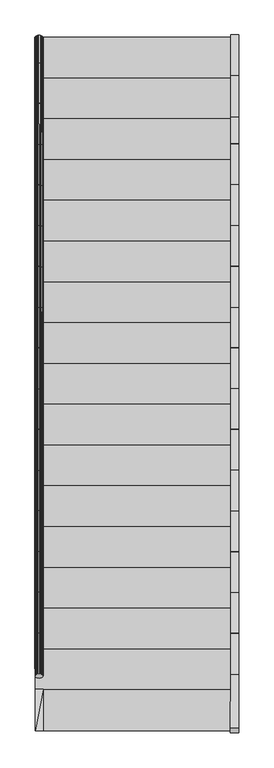
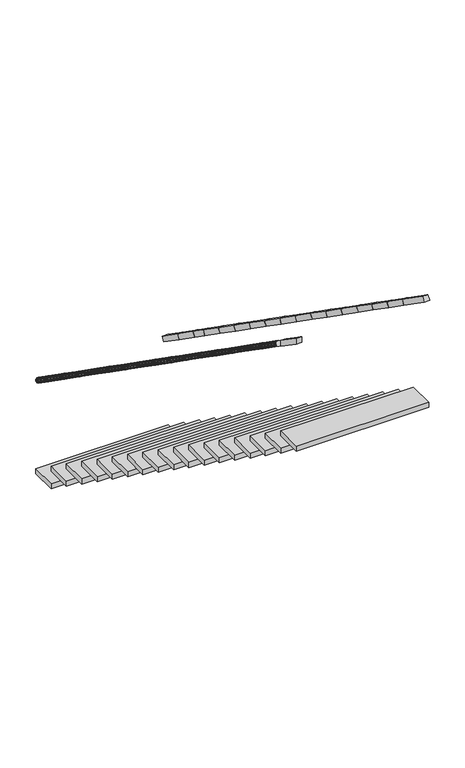
"""IFC4 building model written with IfcOpenShell, lengths in millimetres: stair geometry, 0_3d."""

from ifc_helpers import new_model, si_unit, frame, origin, origin_with_axes, place, context, project, spatial, polyline, outline, extrude, faceted_brep, source, transform, mapped, element, save


def stair_a708374c(model_context):
    return source(origin(), model_context, "Body", "SolidModel", [
        extrude(outline(polyline([(1249.4490496, 514.5019196), (1249.4123204, 264.3787636), (0.5876783, 268.1325506), (0.5509483, 518.0098269), (1249.4490496, 514.5019196)])), frame((0.0, 0.0, 2625.0), z_axis=(0.0, 0.0, 1.0), x_axis=(1.0, 0.0, 0.0)), (0.0, 0.0, 1.0), 50.0),
        extrude(outline(polyline([(8.0820225, -49.3424858), (0.0, 0.0), (301.2464918, 49.3424859), (309.3285142, 1e-07), (8.0820225, -49.3424858)])), frame((1249.9611524, 4001.8916658, 1074.5520464), z_axis=(8.41828832501973e-05, 0.5732803649279318, 0.8193592716881524), x_axis=(-0.1617591834181913, -0.8085607212194018, 0.5657415723464564)), (0.0, 0.0, 1.0), 50.0),
        faceted_brep([(1.4325369, 2844.6597545, 1907.7450176), (0.2083434, 2848.7849185, 1913.6355824), (1.4313241, 2852.9104422, 1919.5261472), (4.9817651, 2856.6324906, 1924.8401024), (10.5121244, 2859.5867237, 1929.0572812), (17.4810521, 2861.4839606, 1931.7648767), (25.2063808, 2862.1384864, 1932.6978505), (32.9319016, 2861.4862317, 1931.7648767), (39.9013867, 2859.5910437, 1929.0572812), (45.4326143, 2856.6384366, 1924.8401024), (48.9841494, 2852.9174321, 1919.5261472), (50.2083429, 2848.7922681, 1913.6355824), (48.9853622, 2844.6667444, 1907.7450176), (45.4349212, 2840.944696, 1902.4310623), (39.9045618, 2837.9904629, 1898.2138835), (32.9356342, 2836.093226, 1895.5062881), (25.2103054, 2835.4387002, 1894.5733142), (17.4847846, 2836.0909549, 1895.5062881), (10.5152995, 2837.9861429, 1898.2138835), (4.9840719, 2840.9387501, 1902.4310623), (0.245074, 2598.9029786, 2088.6355868), (1.4680547, 2603.028502, 2094.5261518), (5.0184957, 2606.7505501, 2099.8401073), (10.548855, 2609.704783, 2104.0572862), (17.5177827, 2611.6020197, 2106.7648818), (25.2431114, 2612.2565455, 2107.6978556), (32.9686322, 2611.6042908, 2106.7648818), (39.9381173, 2609.709103, 2104.0572862), (45.4693449, 2606.7564961, 2099.8401073), (49.02088, 2603.0354919, 2094.5261518), (50.2450735, 2598.9103282, 2088.6355868), (49.0220928, 2594.7848048, 2082.7450218), (45.4716518, 2591.0627567, 2077.4310663), (39.9412924, 2588.1085238, 2073.2138874), (32.9723648, 2586.2112871, 2070.5062918), (25.2470361, 2585.5567613, 2069.573318), (17.5215152, 2586.209016, 2070.5062918), (10.5520301, 2588.1042038, 2073.2138874), (5.0208025, 2591.0568107, 2077.4310663), (1.4692675, 2594.7778149, 2082.7450218)], [[[0, 1, 2, 3, 4, 5, 6, 7, 8, 9, 10, 11, 12, 13, 14, 15, 16, 17, 18, 19]], [[2, 1, 20, 21]], [[3, 2, 21, 22]], [[4, 3, 22, 23]], [[5, 4, 23, 24]], [[6, 5, 24, 25]], [[7, 6, 25, 26]], [[8, 7, 26, 27]], [[9, 8, 27, 28]], [[10, 9, 28, 29]], [[11, 10, 29, 30]], [[12, 11, 30, 31]], [[13, 12, 31, 32]], [[14, 13, 32, 33]], [[15, 14, 33, 34]], [[16, 15, 34, 35]], [[17, 16, 35, 36]], [[18, 17, 36, 37]], [[19, 18, 37, 38]], [[0, 19, 38, 39]], [[1, 0, 39, 20]], [[21, 20, 39, 38, 37, 36, 35, 34, 33, 32, 31, 30, 29, 28, 27, 26, 25, 24, 23, 22]]]),
        extrude(outline(polyline([(1249.5225078, 1014.7482313), (1249.4857787, 764.6250755), (0.5142184, 767.8870744), (0.4774885, 1017.7642932), (1249.5225078, 1014.7482313)])), frame((0.0, 0.0, 2275.0), z_axis=(0.0, 0.0, 1.0), x_axis=(1.0, 0.0, 0.0)), (0.0, 0.0, 1.0), 50.0),
        faceted_brep([(1.4692675, 2594.7778149, 2082.7450218), (0.245074, 2598.9029786, 2088.6355868), (1.4680547, 2603.028502, 2094.5261518), (5.0184957, 2606.7505501, 2099.8401073), (10.548855, 2609.704783, 2104.0572862), (17.5177827, 2611.6020197, 2106.7648818), (25.2431114, 2612.2565455, 2107.6978556), (32.9686322, 2611.6042908, 2106.7648818), (39.9381173, 2609.709103, 2104.0572862), (45.4693449, 2606.7564961, 2099.8401073), (49.02088, 2603.0354919, 2094.5261518), (50.2450735, 2598.9103282, 2088.6355868), (49.0220928, 2594.7848048, 2082.7450218), (45.4716518, 2591.0627567, 2077.4310663), (39.9412924, 2588.1085238, 2073.2138874), (32.9723648, 2586.2112871, 2070.5062918), (25.2470361, 2585.5567613, 2069.573318), (17.5215152, 2586.209016, 2070.5062918), (10.5520301, 2588.1042038, 2073.2138874), (5.0208025, 2591.0568107, 2077.4310663), (0.2818046, 2349.0210098, 2263.6355913), (1.5047853, 2353.1465328, 2269.5261565), (5.0552263, 2356.8685807, 2274.8401122), (10.5855856, 2359.8228133, 2279.0572913), (17.5545133, 2361.7200499, 2281.7648869), (25.279842, 2362.3745756, 2282.6978608), (33.0053628, 2361.722321, 2281.7648869), (39.9748479, 2359.8271333, 2279.0572913), (45.5060756, 2356.8745266, 2274.8401122), (49.0576106, 2353.1535227, 2269.5261565), (50.2818041, 2349.0283594, 2263.6355913), (49.0588234, 2344.9028363, 2257.745026), (45.5083824, 2341.1807885, 2252.4310703), (39.978023, 2338.2265558, 2248.2138912), (33.0090954, 2336.3293193, 2245.5062956), (25.2837667, 2335.6747935, 2244.5733217), (17.5582459, 2336.3270481, 2245.5062956), (10.5887608, 2338.2222359, 2248.2138912), (5.0575331, 2341.1748425, 2252.4310703), (1.5059981, 2344.8958464, 2257.745026)], [[[0, 1, 2, 3, 4, 5, 6, 7, 8, 9, 10, 11, 12, 13, 14, 15, 16, 17, 18, 19]], [[2, 1, 20, 21]], [[3, 2, 21, 22]], [[4, 3, 22, 23]], [[5, 4, 23, 24]], [[6, 5, 24, 25]], [[7, 6, 25, 26]], [[8, 7, 26, 27]], [[9, 8, 27, 28]], [[10, 9, 28, 29]], [[11, 10, 29, 30]], [[12, 11, 30, 31]], [[13, 12, 31, 32]], [[14, 13, 32, 33]], [[15, 14, 33, 34]], [[16, 15, 34, 35]], [[17, 16, 35, 36]], [[18, 17, 36, 37]], [[19, 18, 37, 38]], [[0, 19, 38, 39]], [[1, 0, 39, 20]], [[21, 20, 39, 38, 37, 36, 35, 34, 33, 32, 31, 30, 29, 28, 27, 26, 25, 24, 23, 22]]]),
        extrude(outline(polyline([(8.0820225, -49.3424858), (0.0, 0.0), (301.2464919, 49.3424859), (309.3285143, 1e-07), (8.0820225, -49.3424858)])), frame((1249.7895422, 2833.2364482, 1892.2240093), z_axis=(8.418288334449686e-05, 0.5732803647665086, 0.8193592718010952), x_axis=(-0.16175918336906983, -0.8085607213374504, 0.5657415721917858)), (0.0, 0.0, 1.0), 50.0),
        extrude(outline(polyline([(8.0820225, -49.3424859), (0.0, 0.0), (301.246492, 49.3424859), (309.3285144, 0.0), (8.0820225, -49.3424859)])), frame((1249.679357, 2082.8817614, 2417.2240094), z_axis=(8.418288319098076e-05, 0.5732803645012542, 0.8193592719866855), x_axis=(-0.16175918329309924, -0.8085607215308216, 0.5657415719371407)), (0.0, 0.0, 1.0), 50.0),
        extrude(outline(polyline([(8.0820225, -49.3424859), (0.0, 0.0), (301.2464924, 49.3424859), (309.3285148, 0.0), (8.0820225, -49.3424859)])), frame((1249.495715, 832.2906153, 3292.2240094), z_axis=(8.418288310454991e-05, 0.5732803637766174, 0.8193592724936917), x_axis=(-0.16175918308892365, -0.8085607220586004, 0.565741571241215)), (0.0, 0.0, 1.0), 50.0),
        extrude(outline(polyline([(1249.6326952, 1765.1176979), (1249.5959661, 1514.9945425), (0.4040287, 1517.5186441), (0.3672988, 1767.3957763), (1249.6326952, 1765.1176979)])), frame((0.0, 0.0, 1750.0), z_axis=(0.0, 0.0, 1.0), x_axis=(1.0, 0.0, 0.0)), (0.0, 0.0, 1.0), 50.0),
        faceted_brep([(1.3958063, 3094.5416652, 1732.7450133), (0.1716128, 3098.6668296, 1738.6355779), (1.3945935, 3102.7923536, 1744.5261425), (4.9450345, 3106.5144023, 1749.8400975), (10.4753938, 3109.4686356, 1754.0572762), (17.4443215, 3111.3658726, 1756.7648715), (25.1696502, 3112.0203985, 1757.6978453), (32.895171, 3111.3681438, 1756.7648715), (39.8646561, 3109.4729556, 1754.0572762), (45.3958837, 3106.5203482, 1749.8400975), (48.9474188, 3102.7993435, 1744.5261425), (50.1716122, 3098.6741791, 1738.6355779), (48.9486316, 3094.5486551, 1732.7450133), (45.3981906, 3090.8266064, 1727.4310583), (39.8678312, 3087.8723731, 1723.2138796), (32.8989036, 3085.9751361, 1720.5062843), (25.1735748, 3085.3206102, 1719.5733105), (17.448054, 3085.9728649, 1720.5062843), (10.4785689, 3087.8680531, 1723.2138796), (4.9473413, 3090.8206605, 1727.4310583), (0.2083434, 2848.7849185, 1913.6355824), (1.4313241, 2852.9104422, 1919.5261472), (4.9817651, 2856.6324906, 1924.8401024), (10.5121244, 2859.5867237, 1929.0572812), (17.4810521, 2861.4839606, 1931.7648767), (25.2063808, 2862.1384864, 1932.6978505), (32.9319016, 2861.4862317, 1931.7648767), (39.9013867, 2859.5910437, 1929.0572812), (45.4326143, 2856.6384366, 1924.8401024), (48.9841494, 2852.9174321, 1919.5261472), (50.2083429, 2848.7922681, 1913.6355824), (48.9853622, 2844.6667444, 1907.7450176), (45.4349212, 2840.944696, 1902.4310623), (39.9045618, 2837.9904629, 1898.2138835), (32.9356342, 2836.093226, 1895.5062881), (25.2103054, 2835.4387002, 1894.5733142), (17.4847846, 2836.0909549, 1895.5062881), (10.5152995, 2837.9861429, 1898.2138835), (4.9840719, 2840.9387501, 1902.4310623), (1.4325369, 2844.6597545, 1907.7450176)], [[[0, 1, 2, 3, 4, 5, 6, 7, 8, 9, 10, 11, 12, 13, 14, 15, 16, 17, 18, 19]], [[2, 1, 20, 21]], [[3, 2, 21, 22]], [[4, 3, 22, 23]], [[5, 4, 23, 24]], [[6, 5, 24, 25]], [[7, 6, 25, 26]], [[8, 7, 26, 27]], [[9, 8, 27, 28]], [[10, 9, 28, 29]], [[11, 10, 29, 30]], [[12, 11, 30, 31]], [[13, 12, 31, 32]], [[14, 13, 32, 33]], [[15, 14, 33, 34]], [[16, 15, 34, 35]], [[17, 16, 35, 36]], [[18, 17, 36, 37]], [[19, 18, 37, 38]], [[0, 19, 38, 39]], [[1, 0, 39, 20]], [[21, 20, 39, 38, 37, 36, 35, 34, 33, 32, 31, 30, 29, 28, 27, 26, 25, 24, 23, 22]]]),
        extrude(outline(polyline([(1249.7061535, 2265.3640086), (1249.6694243, 2015.2408533), (0.3305689, 2017.2728797), (0.293839, 2267.1499541), (1249.7061535, 2265.3640086)])), frame((0.0, 0.0, 1400.0), z_axis=(0.0, 0.0, 1.0), x_axis=(1.0, 0.0, 0.0)), (0.0, 0.0, 1.0), 50.0),
        faceted_brep([(1.7263819, 845.6034293, 3307.7450513), (0.5021884, 849.7285907, 3313.6356179), (1.7251691, 853.8541119, 3319.5261845), (5.27561, 857.576158, 3324.8401414), (10.8059694, 860.5303893, 3329.0573215), (17.7748971, 862.4276249, 3331.7649177), (25.5002258, 863.0821504, 3332.6978918), (33.2257466, 862.4298961, 3331.7649177), (40.1952317, 860.5347092, 3329.0573215), (45.7264593, 857.5821039, 3324.8401414), (49.2779944, 853.8611018, 3319.5261845), (50.5021878, 849.7359403, 3313.6356179), (49.2792072, 845.6104192, 3307.7450513), (45.7287662, 841.8883731, 3302.4310944), (40.1984068, 838.9341418, 3298.2139144), (33.2294792, 837.0369061, 3295.5063181), (25.5041504, 836.3823807, 3294.573344), (17.7786296, 837.034635, 3295.5063181), (10.8091445, 838.9298218, 3298.2139144), (5.2779169, 841.8824271, 3302.4310944), (0.538919, 599.84642, 3488.6356224), (1.7618997, 603.9719408, 3494.5261892), (5.3123407, 607.6939866, 3499.8401463), (10.8427001, 610.6482177, 3504.0573265), (17.8116277, 612.5454532, 3506.7649229), (25.5369564, 613.1999786, 3507.697897), (33.2624772, 612.5477243, 3506.7649229), (40.2319623, 610.6525376, 3504.0573265), (45.76319, 607.6999326, 3499.8401463), (49.314725, 603.9789307, 3494.5261892), (50.5389185, 599.8537696, 3488.6356224), (49.3159378, 595.7282487, 3482.7450556), (45.7654968, 592.0062029, 3477.4310985), (40.2351375, 589.0519719, 3473.2139182), (33.2662098, 587.1547364, 3470.5063219), (25.5408811, 586.500211, 3469.5733477), (17.8153603, 587.1524652, 3470.5063219), (10.8458752, 589.0476519, 3473.2139182), (5.3146475, 592.000257, 3477.4310985), (1.7631125, 595.7212589, 3482.7450556)], [[[0, 1, 2, 3, 4, 5, 6, 7, 8, 9, 10, 11, 12, 13, 14, 15, 16, 17, 18, 19]], [[2, 1, 20, 21]], [[3, 2, 21, 22]], [[4, 3, 22, 23]], [[5, 4, 23, 24]], [[6, 5, 24, 25]], [[7, 6, 25, 26]], [[8, 7, 26, 27]], [[9, 8, 27, 28]], [[10, 9, 28, 29]], [[11, 10, 29, 30]], [[12, 11, 30, 31]], [[13, 12, 31, 32]], [[14, 13, 32, 33]], [[15, 14, 33, 34]], [[16, 15, 34, 35]], [[17, 16, 35, 36]], [[18, 17, 36, 37]], [[19, 18, 37, 38]], [[0, 19, 38, 39]], [[1, 0, 39, 20]], [[21, 20, 39, 38, 37, 36, 35, 34, 33, 32, 31, 30, 29, 28, 27, 26, 25, 24, 23, 22]]]),
        faceted_brep([(0.6244082, 14.2556075, 3867.0), (0.5876783, 268.1325506, 3692.0), (50.5877009, 267.9822577, 3692.0), (50.6244323, 14.2555335, 3867.0), (50.5877009, 267.9822577, 3750.0), (0.5876783, 268.1325506, 3750.0), (0.6244082, 14.2556075, 3925.0), (50.6244323, 14.2555335, 3925.0)], [[[0, 1, 2]], [[3, 0, 2]], [[4, 5, 6]], [[7, 4, 6]], [[4, 2, 1, 5]], [[5, 1, 0, 6]], [[6, 0, 3, 7]], [[7, 3, 2, 4]]]),
        extrude(outline(polyline([(8.0820224, -49.3424859), (0.0, 0.0), (301.2464922, 49.3424859), (309.3285146, 0.0), (8.0820224, -49.3424859)])), frame((1249.5691718, 1332.527074, 2942.2240094), z_axis=(8.418288311948242e-05, 0.5732803641088847, 0.8193592722612145), x_axis=(-0.16175918318212845, -0.8085607218166563, 0.5657415715603531)), (0.0, 0.0, 1.0), 50.0),
        extrude(outline(polyline([(1.2235871, -7.1914683), (0.0, 0.0), (1.2235871, 7.1914683), (4.7745752, 13.6789855), (10.3053687, 18.8275083), (17.2745752, 22.1330635), (25.0, 23.2720802), (32.7254248, 22.1330635), (39.6946313, 18.8275084), (45.2254248, 13.6789855), (48.7764129, 7.1914683), (50.0, 0.0), (48.7764129, -7.1914683), (45.2254249, -13.6789854), (39.6946313, -18.8275083), (32.7254249, -22.1330635), (25.0, -23.2720802), (17.2745751, -22.1330634), (10.3053687, -18.8275083), (4.7745751, -13.6789855), (1.2235871, -7.1914683)])), frame((0.0, 4266.1655097, 921.0), z_axis=(0.00012040167666258672, -0.8191044431453997, 0.5736443991907366), x_axis=(0.9999999891966984, 0.00014699184745837235, 0.0)), (0.0, 0.0, 1.0), 205.067042),
        extrude(outline(polyline([(1249.8897991, 3515.9797843), (1249.85307, 3265.8566293), (0.1469195, 3266.6579632), (0.1101896, 3516.5348933), (1249.8897991, 3515.9797843)])), frame((0.0, 0.0, 525.0), z_axis=(0.0, 0.0, 1.0), x_axis=(1.0, 0.0, 0.0)), (0.0, 0.0, 1.0), 50.0),
        extrude(outline(polyline([(1249.8163409, 3015.7334742), (1249.7796117, 2765.610319), (0.2203792, 2766.9040165), (0.1836493, 3016.7810043), (1249.8163409, 3015.7334742)])), frame((0.0, 0.0, 875.0), z_axis=(0.0, 0.0, 1.0), x_axis=(1.0, 0.0, 0.0)), (0.0, 0.0, 1.0), 50.0),
        extrude(outline(polyline([(1249.9999865, 4266.3492495), (1249.9632574, 4016.2260945), (0.0367299, 4016.2886665), (0.0, 4266.1655097), (1249.9999865, 4266.3492495)])), origin_with_axes(), (0.0, 0.0, 1.0), 50.0),
        faceted_brep([(1.5794593, 1845.1318228, 2607.7450345), (0.3552659, 1849.2569855, 2613.6356001), (1.5782465, 1853.3825079, 2619.5261658), (5.1286875, 1857.1045552, 2624.8401219), (10.6590469, 1860.0587874, 2629.0573013), (17.6279745, 1861.9560236, 2631.7648972), (25.3533033, 1862.6105493, 2632.6978712), (33.0788241, 1861.9582948, 2631.7648972), (40.0483092, 1860.0631074, 2629.0573013), (45.5795368, 1857.1105012, 2624.8401219), (49.1310718, 1853.3894978, 2619.5261658), (50.3552653, 1849.2643351, 2613.6356001), (49.1322846, 1845.1388127, 2607.7450345), (45.5818436, 1841.4167654, 2602.4310784), (40.0514843, 1838.4625333, 2598.213899), (33.0825566, 1836.565297, 2595.5063031), (25.3572279, 1835.9107713, 2594.5733291), (17.6317071, 1836.5630258, 2595.5063031), (10.662222, 1838.4582133, 2598.213899), (5.1309944, 1841.4108195, 2602.4310784), (0.3919965, 1599.3749301, 2788.6356046), (1.6149772, 1603.5004522, 2794.5261705), (5.1654181, 1607.2224992, 2799.8401268), (10.6957775, 1610.1767311, 2804.0573064), (17.6647052, 1612.0739672, 2806.7649023), (25.3900339, 1612.7284928, 2807.6978763), (33.1155547, 1612.0762384, 2806.7649023), (40.0850398, 1610.1810511, 2804.0573064), (45.6162674, 1607.2284451, 2799.8401268), (49.1678025, 1603.5074421, 2794.5261705), (50.3919959, 1599.3822797, 2788.6356046), (49.1690153, 1595.2567576, 2782.7450387), (45.6185743, 1591.5347106, 2777.4310824), (40.0882149, 1588.5804787, 2773.2139028), (33.1192873, 1586.6832425, 2770.5063068), (25.3939585, 1586.0287169, 2769.5733329), (17.6684377, 1586.6809714, 2770.5063068), (10.6989526, 1588.5761587, 2773.2139028), (5.167725, 1591.5287647, 2777.4310824), (1.6161899, 1595.2497677, 2782.7450387)], [[[0, 1, 2, 3, 4, 5, 6, 7, 8, 9, 10, 11, 12, 13, 14, 15, 16, 17, 18, 19]], [[2, 1, 20, 21]], [[3, 2, 21, 22]], [[4, 3, 22, 23]], [[5, 4, 23, 24]], [[6, 5, 24, 25]], [[7, 6, 25, 26]], [[8, 7, 26, 27]], [[9, 8, 27, 28]], [[10, 9, 28, 29]], [[11, 10, 29, 30]], [[12, 11, 30, 31]], [[13, 12, 31, 32]], [[14, 13, 32, 33]], [[15, 14, 33, 34]], [[16, 15, 34, 35]], [[17, 16, 35, 36]], [[18, 17, 36, 37]], [[19, 18, 37, 38]], [[0, 19, 38, 39]], [[1, 0, 39, 20]], [[21, 20, 39, 38, 37, 36, 35, 34, 33, 32, 31, 30, 29, 28, 27, 26, 25, 24, 23, 22]]]),
        faceted_brep([(1.2856145, 3844.1872239, 1207.7450006), (0.061421, 3848.3123892, 1213.6355645), (1.2844017, 3852.4379142, 1219.5261284), (4.8348427, 3856.1599637, 1224.8400829), (10.365202, 3859.1141977, 1229.057261), (17.3341297, 3861.0114352, 1231.7648561), (25.0594584, 3861.6659612, 1232.6978297), (32.7849792, 3861.0137063, 1231.7648561), (39.7544643, 3859.1185177, 1229.057261), (45.2856919, 3856.1659097, 1224.8400829), (48.837227, 3852.444904, 1219.5261284), (50.0614205, 3848.3197388, 1213.6355645), (48.8384398, 3844.1942138, 1207.7450006), (45.2879988, 3840.4721642, 1202.4310462), (39.7576394, 3837.5179302, 1198.213868), (32.7887118, 3835.6206928, 1195.506273), (25.0633831, 3834.9661667, 1194.5732993), (17.3378622, 3835.6184216, 1195.506273), (10.3683771, 3837.5136102, 1198.213868), (4.8371495, 3840.4662183, 1202.4310462), (0.0981516, 3598.4305649, 1388.635569), (1.3211323, 3602.5560896, 1394.5261331), (4.8715733, 3606.2781388, 1399.8400878), (10.4019326, 3609.2323726, 1404.0572661), (17.3708603, 3611.1296099, 1406.7648612), (25.096189, 3611.7841359, 1407.6978349), (32.8217098, 3611.1318811, 1406.7648612), (39.7911949, 3609.2366926, 1404.0572661), (45.3224225, 3606.2840848, 1399.8400878), (48.8739576, 3602.5630794, 1394.5261331), (50.0981511, 3598.4379145, 1388.635569), (48.8751704, 3594.3123898, 1382.7450049), (45.3247294, 3590.5903405, 1377.4310502), (39.79437, 3587.6361067, 1373.2138719), (32.8254424, 3585.7388695, 1370.5062768), (25.1001137, 3585.0843435, 1369.5733031), (17.3745928, 3585.7365983, 1370.5062768), (10.4051077, 3587.6317868, 1373.2138719), (4.8738801, 3590.5843946, 1377.4310502), (1.3223451, 3594.3053999, 1382.7450049)], [[[0, 1, 2, 3, 4, 5, 6, 7, 8, 9, 10, 11, 12, 13, 14, 15, 16, 17, 18, 19]], [[2, 1, 20, 21]], [[3, 2, 21, 22]], [[4, 3, 22, 23]], [[5, 4, 23, 24]], [[6, 5, 24, 25]], [[7, 6, 25, 26]], [[8, 7, 26, 27]], [[9, 8, 27, 28]], [[10, 9, 28, 29]], [[11, 10, 29, 30]], [[12, 11, 30, 31]], [[13, 12, 31, 32]], [[14, 13, 32, 33]], [[15, 14, 33, 34]], [[16, 15, 34, 35]], [[17, 16, 35, 36]], [[18, 17, 36, 37]], [[19, 18, 37, 38]], [[0, 19, 38, 39]], [[1, 0, 39, 20]], [[21, 20, 39, 38, 37, 36, 35, 34, 33, 32, 31, 30, 29, 28, 27, 26, 25, 24, 23, 22]]]),
        faceted_brep([(1.6896512, 1095.4855709, 3132.7450471), (0.4654577, 1099.6107327, 3138.6356135), (1.6884384, 1103.7362542, 3144.5261798), (5.2388794, 1107.4583006, 3149.8401365), (10.7692388, 1110.4125321, 3154.0573164), (17.7381664, 1112.3097679, 3156.7649126), (25.4634951, 1112.9642934, 3157.6978867), (33.189016, 1112.312039, 3156.7649126), (40.1585011, 1110.416852, 3154.0573164), (45.6897287, 1107.4642465, 3149.8401365), (49.2412637, 1103.743244, 3144.5261798), (50.4654572, 1099.6180823, 3138.6356135), (49.2424765, 1095.4925608, 3132.7450471), (45.6920355, 1091.7705144, 3127.4310904), (40.1616762, 1088.8162829, 3123.2139105), (33.1927485, 1086.9190471, 3120.5063144), (25.4674198, 1086.2645216, 3119.5733403), (17.741899, 1086.916776, 3120.5063144), (10.7724139, 1088.811963, 3123.2139105), (5.2411863, 1091.7645685, 3127.4310904), (0.5021884, 849.7285907, 3313.6356179), (1.7251691, 853.8541119, 3319.5261845), (5.27561, 857.576158, 3324.8401414), (10.8059694, 860.5303893, 3329.0573215), (17.7748971, 862.4276249, 3331.7649177), (25.5002258, 863.0821504, 3332.6978918), (33.2257466, 862.4298961, 3331.7649177), (40.1952317, 860.5347092, 3329.0573215), (45.7264593, 857.5821039, 3324.8401414), (49.2779944, 853.8611018, 3319.5261845), (50.5021878, 849.7359403, 3313.6356179), (49.2792072, 845.6104192, 3307.7450513), (45.7287662, 841.8883731, 3302.4310944), (40.1984068, 838.9341418, 3298.2139144), (33.2294792, 837.0369061, 3295.5063181), (25.5041504, 836.3823807, 3294.573344), (17.7786296, 837.034635, 3295.5063181), (10.8091445, 838.9298218, 3298.2139144), (5.2779169, 841.8824271, 3302.4310944), (1.7263819, 845.6034293, 3307.7450513)], [[[0, 1, 2, 3, 4, 5, 6, 7, 8, 9, 10, 11, 12, 13, 14, 15, 16, 17, 18, 19]], [[2, 1, 20, 21]], [[3, 2, 21, 22]], [[4, 3, 22, 23]], [[5, 4, 23, 24]], [[6, 5, 24, 25]], [[7, 6, 25, 26]], [[8, 7, 26, 27]], [[9, 8, 27, 28]], [[10, 9, 28, 29]], [[11, 10, 29, 30]], [[12, 11, 30, 31]], [[13, 12, 31, 32]], [[14, 13, 32, 33]], [[15, 14, 33, 34]], [[16, 15, 34, 35]], [[17, 16, 35, 36]], [[18, 17, 36, 37]], [[19, 18, 37, 38]], [[0, 19, 38, 39]], [[1, 0, 39, 20]], [[21, 20, 39, 38, 37, 36, 35, 34, 33, 32, 31, 30, 29, 28, 27, 26, 25, 24, 23, 22]]]),
        faceted_brep([(1.5059981, 2344.8958464, 2257.745026), (0.2818046, 2349.0210098, 2263.6355913), (1.5047853, 2353.1465328, 2269.5261565), (5.0552263, 2356.8685807, 2274.8401122), (10.5855856, 2359.8228133, 2279.0572913), (17.5545133, 2361.7200499, 2281.7648869), (25.279842, 2362.3745756, 2282.6978608), (33.0053628, 2361.722321, 2281.7648869), (39.9748479, 2359.8271333, 2279.0572913), (45.5060756, 2356.8745266, 2274.8401122), (49.0576106, 2353.1535227, 2269.5261565), (50.2818041, 2349.0283594, 2263.6355913), (49.0588234, 2344.9028363, 2257.745026), (45.5083824, 2341.1807885, 2252.4310703), (39.978023, 2338.2265558, 2248.2138912), (33.0090954, 2336.3293193, 2245.5062956), (25.2837667, 2335.6747935, 2244.5733217), (17.5582459, 2336.3270481, 2245.5062956), (10.5887608, 2338.2222359, 2248.2138912), (5.0575331, 2341.1748425, 2252.4310703), (0.3185352, 2099.1390121, 2438.6355957), (1.5415159, 2103.2645348, 2444.5261612), (5.0919569, 2106.9865824, 2449.8401171), (10.6223163, 2109.9408148, 2454.0572963), (17.5912439, 2111.8380512, 2456.7648921), (25.3165726, 2112.4925769, 2457.697866), (33.0420935, 2111.8403223, 2456.7648921), (40.0115786, 2109.9451348, 2454.0572963), (45.5428062, 2106.9925283, 2449.8401171), (49.0943412, 2103.2715247, 2444.5261612), (50.3185347, 2099.1463617, 2438.6355957), (49.095554, 2095.0208389, 2432.7450302), (45.545113, 2091.2987914, 2427.4310744), (40.0147537, 2088.344559, 2423.2138951), (33.045826, 2086.4473226, 2420.5062993), (25.3204973, 2085.7927969, 2419.5733254), (17.5949765, 2086.4450514, 2420.5062993), (10.6254914, 2088.340239, 2423.2138951), (5.0942637, 2091.2928454, 2427.4310744), (1.5427287, 2095.0138491, 2432.7450302)], [[[0, 1, 2, 3, 4, 5, 6, 7, 8, 9, 10, 11, 12, 13, 14, 15, 16, 17, 18, 19]], [[2, 1, 20, 21]], [[3, 2, 21, 22]], [[4, 3, 22, 23]], [[5, 4, 23, 24]], [[6, 5, 24, 25]], [[7, 6, 25, 26]], [[8, 7, 26, 27]], [[9, 8, 27, 28]], [[10, 9, 28, 29]], [[11, 10, 29, 30]], [[12, 11, 30, 31]], [[13, 12, 31, 32]], [[14, 13, 32, 33]], [[15, 14, 33, 34]], [[16, 15, 34, 35]], [[17, 16, 35, 36]], [[18, 17, 36, 37]], [[19, 18, 37, 38]], [[0, 19, 38, 39]], [[1, 0, 39, 20]], [[21, 20, 39, 38, 37, 36, 35, 34, 33, 32, 31, 30, 29, 28, 27, 26, 25, 24, 23, 22]]]),
        extrude(outline(polyline([(8.0820224, -49.3424859), (0.0, 0.0), (301.2464923, 49.3424859), (309.3285147, 0.0), (8.0820224, -49.3424859)])), frame((1249.5324434, 1082.4088447, 3117.2240094), z_axis=(8.4182883083192e-05, 0.5732803639497914, 0.8193592723725271), x_axis=(-0.16175918313745635, -0.8085607219325107, 0.5657415714075466)), (0.0, 0.0, 1.0), 50.0),
        faceted_brep([(1.6529206, 1345.3676837, 2957.7450429), (0.4287271, 1349.4928458, 2963.635609), (1.6517078, 1353.6183676, 2969.5261752), (5.2021488, 1357.3404143, 2974.8401317), (10.7325081, 1360.294646, 2979.0573114), (17.7014358, 1362.191882, 2981.7649075), (25.4267645, 1362.8464075, 2982.6978815), (33.1522853, 1362.1941531, 2981.7649075), (40.1217704, 1360.298966, 2979.0573114), (45.6529981, 1357.3463602, 2974.8401317), (49.2045331, 1353.6253575, 2969.5261752), (50.4287266, 1349.5001954, 2963.635609), (49.2057459, 1345.3746736, 2957.7450429), (45.6553049, 1341.6526269, 2952.4310864), (40.1249455, 1338.6983952, 2948.2139067), (33.1560179, 1336.8011593, 2945.5063106), (25.4306892, 1336.1466337, 2944.5733366), (17.7051683, 1336.7988881, 2945.5063106), (10.7356832, 1338.6940752, 2948.2139067), (5.2044556, 1341.646681, 2952.4310864), (0.4654577, 1099.6107327, 3138.6356135), (1.6884384, 1103.7362542, 3144.5261798), (5.2388794, 1107.4583006, 3149.8401365), (10.7692388, 1110.4125321, 3154.0573164), (17.7381664, 1112.3097679, 3156.7649126), (25.4634951, 1112.9642934, 3157.6978867), (33.189016, 1112.312039, 3156.7649126), (40.1585011, 1110.416852, 3154.0573164), (45.6897287, 1107.4642465, 3149.8401365), (49.2412637, 1103.743244, 3144.5261798), (50.4654572, 1099.6180823, 3138.6356135), (49.2424765, 1095.4925608, 3132.7450471), (45.6920355, 1091.7705144, 3127.4310904), (40.1616762, 1088.8162829, 3123.2139105), (33.1927485, 1086.9190471, 3120.5063144), (25.4674198, 1086.2645216, 3119.5733403), (17.741899, 1086.916776, 3120.5063144), (10.7724139, 1088.811963, 3123.2139105), (5.2411863, 1091.7645685, 3127.4310904), (1.6896512, 1095.4855709, 3132.7450471)], [[[0, 1, 2, 3, 4, 5, 6, 7, 8, 9, 10, 11, 12, 13, 14, 15, 16, 17, 18, 19]], [[2, 1, 20, 21]], [[3, 2, 21, 22]], [[4, 3, 22, 23]], [[5, 4, 23, 24]], [[6, 5, 24, 25]], [[7, 6, 25, 26]], [[8, 7, 26, 27]], [[9, 8, 27, 28]], [[10, 9, 28, 29]], [[11, 10, 29, 30]], [[12, 11, 30, 31]], [[13, 12, 31, 32]], [[14, 13, 32, 33]], [[15, 14, 33, 34]], [[16, 15, 34, 35]], [[17, 16, 35, 36]], [[18, 17, 36, 37]], [[19, 18, 37, 38]], [[0, 19, 38, 39]], [[1, 0, 39, 20]], [[21, 20, 39, 38, 37, 36, 35, 34, 33, 32, 31, 30, 29, 28, 27, 26, 25, 24, 23, 22]]]),
        extrude(outline(polyline([(8.0820225, -49.3424859), (0.0, 0.0), (301.2464922, 49.3424859), (309.3285146, 0.0), (8.0820225, -49.3424859)])), frame((1249.6059002, 1582.6453033, 2767.2240094), z_axis=(8.418288318234878e-05, 0.5732803642537855, 0.8193592721598316), x_axis=(-0.1617591832231551, -0.808560721711089, 0.5657415716995001)), (0.0, 0.0, 1.0), 50.0),
        extrude(outline(polyline([(11.8336015, -48.5794799), (0.0, 0.0), (199.4292167, 48.57948), (211.2628181, 0.0), (11.8336015, -48.5794799)])), frame((1249.924424, 3751.773437, 1249.5520464), z_axis=(8.418288319610166e-05, 0.5732803649196659, 0.8193592716939356), x_axis=(-0.23678892715388222, -0.7960461843199325, 0.5569932462848984)), (0.0, 0.0, 1.0), 50.0),
        extrude(outline(polyline([(8.0820225, -49.3424858), (0.0, 0.0), (301.2464919, 49.3424859), (309.3285143, 1e-07), (8.0820225, -49.3424858)])), frame((1249.7528138, 2583.1182193, 2067.2240093), z_axis=(8.418288341734137e-05, 0.5732803646922456, 0.8193592718530548), x_axis=(-0.16175918334768244, -0.8085607213915934, 0.5657415721205195)), (0.0, 0.0, 1.0), 50.0),
        extrude(outline(polyline([(1249.85307, 3265.8566293), (1249.8163409, 3015.7334742), (0.1836493, 3016.7810043), (0.1469195, 3266.6579632), (1249.85307, 3265.8566293)])), frame((0.0, 0.0, 700.0), z_axis=(0.0, 0.0, 1.0), x_axis=(1.0, 0.0, 0.0)), (0.0, 0.0, 1.0), 50.0),
        extrude(outline(polyline([(1249.7796117, 2765.610319), (1249.7428826, 2515.4871638), (0.2571091, 2517.0269998), (0.2203792, 2766.9040165), (1249.7796117, 2765.610319)])), frame((0.0, 0.0, 1050.0), z_axis=(0.0, 0.0, 1.0), x_axis=(1.0, 0.0, 0.0)), (0.0, 0.0, 1.0), 50.0),
        extrude(outline(polyline([(1249.9632574, 4016.2260945), (1249.9265282, 3766.1029394), (0.0734597, 3766.4117944), (0.0367299, 4016.2886665), (1249.9632574, 4016.2260945)])), frame((0.0, 0.0, 175.0), z_axis=(0.0, 0.0, 1.0), x_axis=(1.0, 0.0, 0.0)), (0.0, 0.0, 1.0), 50.0),
        faceted_brep([(1.3223451, 3594.3053999, 1382.7450049), (0.0981516, 3598.4305649, 1388.635569), (1.3211323, 3602.5560896, 1394.5261331), (4.8715733, 3606.2781388, 1399.8400878), (10.4019326, 3609.2323726, 1404.0572661), (17.3708603, 3611.1296099, 1406.7648612), (25.096189, 3611.7841359, 1407.6978349), (32.8217098, 3611.1318811, 1406.7648612), (39.7911949, 3609.2366926, 1404.0572661), (45.3224225, 3606.2840848, 1399.8400878), (48.8739576, 3602.5630794, 1394.5261331), (50.0981511, 3598.4379145, 1388.635569), (48.8751704, 3594.3123898, 1382.7450049), (45.3247294, 3590.5903405, 1377.4310502), (39.79437, 3587.6361067, 1373.2138719), (32.8254424, 3585.7388695, 1370.5062768), (25.1001137, 3585.0843435, 1369.5733031), (17.3745928, 3585.7365983, 1370.5062768), (10.4051077, 3587.6317868, 1373.2138719), (4.8738801, 3590.5843946, 1377.4310502), (0.1348822, 3348.5487117, 1563.6355734), (1.3578629, 3352.674236, 1569.5261378), (4.9083039, 3356.396285, 1574.8400927), (10.4386632, 3359.3505186, 1579.0572711), (17.4075909, 3361.2477557, 1581.7648664), (25.1329196, 3361.9022817, 1582.6978401), (32.8584404, 3361.2500269, 1581.7648664), (39.8279255, 3359.3548385, 1579.0572711), (45.3591531, 3356.402231, 1574.8400927), (48.9106882, 3352.6812259, 1569.5261378), (50.1348816, 3348.5560613, 1563.6355734), (48.911901, 3344.4305369, 1557.7450091), (45.36146, 3340.7084879, 1552.4310542), (39.8311006, 3337.7542544, 1548.2138758), (32.862173, 3335.8570172, 1545.5062805), (25.1368442, 3335.2024913, 1544.5733068), (17.4113234, 3335.8547461, 1545.5062805), (10.4418383, 3337.7499344, 1548.2138758), (4.9106107, 3340.702542, 1552.4310542), (1.3590757, 3344.423547, 1557.7450091)], [[[0, 1, 2, 3, 4, 5, 6, 7, 8, 9, 10, 11, 12, 13, 14, 15, 16, 17, 18, 19]], [[2, 1, 20, 21]], [[3, 2, 21, 22]], [[4, 3, 22, 23]], [[5, 4, 23, 24]], [[6, 5, 24, 25]], [[7, 6, 25, 26]], [[8, 7, 26, 27]], [[9, 8, 27, 28]], [[10, 9, 28, 29]], [[11, 10, 29, 30]], [[12, 11, 30, 31]], [[13, 12, 31, 32]], [[14, 13, 32, 33]], [[15, 14, 33, 34]], [[16, 15, 34, 35]], [[17, 16, 35, 36]], [[18, 17, 36, 37]], [[19, 18, 37, 38]], [[0, 19, 38, 39]], [[1, 0, 39, 20]], [[21, 20, 39, 38, 37, 36, 35, 34, 33, 32, 31, 30, 29, 28, 27, 26, 25, 24, 23, 22]]]),
        extrude(outline(polyline([(8.0820225, -49.3424858), (0.0, 0.0), (301.2464917, 49.3424859), (309.3285142, 1e-07), (8.0820225, -49.3424858)])), frame((1249.9978808, 4252.0098945, 899.5520464), z_axis=(8.418288330599988e-05, 0.5732803649220624, 0.8193592716922591), x_axis=(-0.16175918341661352, -0.8085607212236612, 0.5657415723408199)), (0.0, 0.0, 1.0), 50.0),
        extrude(outline(polyline([(1249.5959661, 1514.9945425), (1249.5592369, 1264.8713869), (0.4407586, 1267.6414831), (0.4040287, 1517.5186441), (1249.5959661, 1514.9945425)])), frame((0.0, 0.0, 1925.0), z_axis=(0.0, 0.0, 1.0), x_axis=(1.0, 0.0, 0.0)), (0.0, 0.0, 1.0), 50.0),
        extrude(outline(polyline([(8.0820225, -49.3424858), (0.0, 0.0), (301.2464918, 49.3424859), (309.3285142, 1e-07), (8.0820225, -49.3424858)])), frame((1249.8262706, 3083.354677, 1717.2240093), z_axis=(8.418288321802858e-05, 0.5732803648266481, 0.8193592717590175), x_axis=(-0.16175918338648482, -0.8085607212935979, 0.5657415722494806)), (0.0, 0.0, 1.0), 50.0),
        faceted_brep([(1.6161899, 1595.2497677, 2782.7450387), (0.3919965, 1599.3749301, 2788.6356046), (1.6149772, 1603.5004522, 2794.5261705), (5.1654181, 1607.2224992, 2799.8401268), (10.6957775, 1610.1767311, 2804.0573064), (17.6647052, 1612.0739672, 2806.7649023), (25.3900339, 1612.7284928, 2807.6978763), (33.1155547, 1612.0762384, 2806.7649023), (40.0850398, 1610.1810511, 2804.0573064), (45.6162674, 1607.2284451, 2799.8401268), (49.1678025, 1603.5074421, 2794.5261705), (50.3919959, 1599.3822797, 2788.6356046), (49.1690153, 1595.2567576, 2782.7450387), (45.6185743, 1591.5347106, 2777.4310824), (40.0882149, 1588.5804787, 2773.2139028), (33.1192873, 1586.6832425, 2770.5063068), (25.3939585, 1586.0287169, 2769.5733329), (17.6684377, 1586.6809714, 2770.5063068), (10.6989526, 1588.5761587, 2773.2139028), (5.167725, 1591.5287647, 2777.4310824), (0.4287271, 1349.4928458, 2963.635609), (1.6517078, 1353.6183676, 2969.5261752), (5.2021488, 1357.3404143, 2974.8401317), (10.7325081, 1360.294646, 2979.0573114), (17.7014358, 1362.191882, 2981.7649075), (25.4267645, 1362.8464075, 2982.6978815), (33.1522853, 1362.1941531, 2981.7649075), (40.1217704, 1360.298966, 2979.0573114), (45.6529981, 1357.3463602, 2974.8401317), (49.2045331, 1353.6253575, 2969.5261752), (50.4287266, 1349.5001954, 2963.635609), (49.2057459, 1345.3746736, 2957.7450429), (45.6553049, 1341.6526269, 2952.4310864), (40.1249455, 1338.6983952, 2948.2139067), (33.1560179, 1336.8011593, 2945.5063106), (25.4306892, 1336.1466337, 2944.5733366), (17.7051683, 1336.7988881, 2945.5063106), (10.7356832, 1338.6940752, 2948.2139067), (5.2044556, 1341.646681, 2952.4310864), (1.6529206, 1345.3676837, 2957.7450429)], [[[0, 1, 2, 3, 4, 5, 6, 7, 8, 9, 10, 11, 12, 13, 14, 15, 16, 17, 18, 19]], [[2, 1, 20, 21]], [[3, 2, 21, 22]], [[4, 3, 22, 23]], [[5, 4, 23, 24]], [[6, 5, 24, 25]], [[7, 6, 25, 26]], [[8, 7, 26, 27]], [[9, 8, 27, 28]], [[10, 9, 28, 29]], [[11, 10, 29, 30]], [[12, 11, 30, 31]], [[13, 12, 31, 32]], [[14, 13, 32, 33]], [[15, 14, 33, 34]], [[16, 15, 34, 35]], [[17, 16, 35, 36]], [[18, 17, 36, 37]], [[19, 18, 37, 38]], [[0, 19, 38, 39]], [[1, 0, 39, 20]], [[21, 20, 39, 38, 37, 36, 35, 34, 33, 32, 31, 30, 29, 28, 27, 26, 25, 24, 23, 22]]]),
        faceted_brep([(1.7631125, 595.7212589, 3482.7450556), (0.538919, 599.84642, 3488.6356224), (1.7618997, 603.9719408, 3494.5261892), (5.3123407, 607.6939866, 3499.8401463), (10.8427001, 610.6482177, 3504.0573265), (17.8116277, 612.5454532, 3506.7649229), (25.5369564, 613.1999786, 3507.697897), (33.2624772, 612.5477243, 3506.7649229), (40.2319623, 610.6525376, 3504.0573265), (45.76319, 607.6999326, 3499.8401463), (49.314725, 603.9789307, 3494.5261892), (50.5389185, 599.8537696, 3488.6356224), (49.3159378, 595.7282487, 3482.7450556), (45.7654968, 592.0062029, 3477.4310985), (40.2351375, 589.0519719, 3473.2139182), (33.2662098, 587.1547364, 3470.5063219), (25.5408811, 586.500211, 3469.5733477), (17.8153603, 587.1524652, 3470.5063219), (10.8458752, 589.0476519, 3473.2139182), (5.3146475, 592.000257, 3477.4310985), (0.5756497, 349.9642204, 3663.6356268), (1.7986304, 354.0897409, 3669.5261938), (5.3490713, 357.8117864, 3674.8401511), (10.8794307, 360.7660172, 3679.0573315), (17.8483583, 362.6632526, 3681.764928), (25.5736871, 363.317778, 3682.6979021), (33.2992079, 362.6655238, 3681.764928), (40.268693, 360.7703372, 3679.0573315), (45.7999206, 357.8177324, 3674.8401511), (49.3514557, 354.0967308, 3669.5261938), (50.5756491, 349.97157, 3663.6356268), (49.3526684, 345.8460495, 3657.7450598), (45.8022275, 342.1240039, 3652.4311025), (40.2718681, 339.1697731, 3648.2139221), (33.3029405, 337.2725377, 3645.5063256), (25.5776117, 336.6180124, 3644.5733514), (17.8520909, 337.2702666, 3645.5063256), (10.8826058, 339.1654531, 3648.2139221), (5.3513782, 342.118058, 3652.4311025), (1.7998431, 345.8390596, 3657.7450598)], [[[0, 1, 2, 3, 4, 5, 6, 7, 8, 9, 10, 11, 12, 13, 14, 15, 16, 17, 18, 19]], [[2, 1, 20, 21]], [[3, 2, 21, 22]], [[4, 3, 22, 23]], [[5, 4, 23, 24]], [[6, 5, 24, 25]], [[7, 6, 25, 26]], [[8, 7, 26, 27]], [[9, 8, 27, 28]], [[10, 9, 28, 29]], [[11, 10, 29, 30]], [[12, 11, 30, 31]], [[13, 12, 31, 32]], [[14, 13, 32, 33]], [[15, 14, 33, 34]], [[16, 15, 34, 35]], [[17, 16, 35, 36]], [[18, 17, 36, 37]], [[19, 18, 37, 38]], [[0, 19, 38, 39]], [[1, 0, 39, 20]], [[21, 20, 39, 38, 37, 36, 35, 34, 33, 32, 31, 30, 29, 28, 27, 26, 25, 24, 23, 22]]]),
        extrude(outline(polyline([(8.0820225, -49.3424858), (0.0, 0.0), (301.2464918, 49.3424859), (309.3285142, 1e-07), (8.0820225, -49.3424858)])), frame((1249.862999, 3333.4729058, 1542.2240093), z_axis=(8.418288315989453e-05, 0.5732803648726768, 0.8193592717268128), x_axis=(-0.1617591834003618, -0.8085607212599576, 0.5657415722935918)), (0.0, 0.0, 1.0), 50.0),
        extrude(outline(polyline([(1249.5592369, 1264.8713869), (1249.5225078, 1014.7482313), (0.4774885, 1017.7642932), (0.4407586, 1267.6414831), (1249.5592369, 1264.8713869)])), frame((0.0, 0.0, 2100.0), z_axis=(0.0, 0.0, 1.0), x_axis=(1.0, 0.0, 0.0)), (0.0, 0.0, 1.0), 50.0),
        extrude(outline(polyline([(1249.7428826, 2515.4871638), (1249.7061535, 2265.3640086), (0.293839, 2267.1499541), (0.2571091, 2517.0269998), (1249.7428826, 2515.4871638)])), frame((0.0, 0.0, 1225.0), z_axis=(0.0, 0.0, 1.0), x_axis=(1.0, 0.0, 0.0)), (0.0, 0.0, 1.0), 50.0),
        extrude(outline(polyline([(8.0820224, -49.3424858), (0.0, 0.0), (301.2464917, 49.3424859), (309.3285142, 1e-07), (8.0820224, -49.3424858)])), frame((1249.8997274, 3583.5911345, 1367.2240093), z_axis=(8.418288314084033e-05, 0.5732803649046162, 0.8193592717044657), x_axis=(-0.1617591834100128, -0.8085607212366094, 0.5657415723242016)), (0.0, 0.0, 1.0), 50.0),
        extrude(outline(polyline([(1249.4857787, 764.6250755), (1249.4490496, 514.5019196), (0.5509483, 518.0098269), (0.5142184, 767.8870744), (1249.4857787, 764.6250755)])), frame((0.0, 0.0, 2450.0), z_axis=(0.0, 0.0, 1.0), x_axis=(1.0, 0.0, 0.0)), (0.0, 0.0, 1.0), 50.0),
        extrude(outline(polyline([(1249.6694243, 2015.2408533), (1249.6326952, 1765.1176979), (0.3672988, 1767.3957763), (0.3305689, 2017.2728797), (1249.6694243, 2015.2408533)])), frame((0.0, 0.0, 1575.0), z_axis=(0.0, 0.0, 1.0), x_axis=(1.0, 0.0, 0.0)), (0.0, 0.0, 1.0), 50.0),
        extrude(outline(polyline([(8.0820225, -49.3424859), (0.0, 0.0), (301.246492, 49.3424859), (309.3285145, 0.0), (8.0820225, -49.3424859)])), frame((1249.6426286, 1832.7635324, 2592.2240094), z_axis=(8.41828831730923e-05, 0.5732803643846047, 0.8193592720683017), x_axis=(-0.16175918326000965, -0.8085607216158117, 0.5657415718251334)), (0.0, 0.0, 1.0), 50.0),
        faceted_brep([(1.5427287, 2095.0138491, 2432.7450302), (0.3185352, 2099.1390121, 2438.6355957), (1.5415159, 2103.2645348, 2444.5261612), (5.0919569, 2106.9865824, 2449.8401171), (10.6223163, 2109.9408148, 2454.0572963), (17.5912439, 2111.8380512, 2456.7648921), (25.3165726, 2112.4925769, 2457.697866), (33.0420935, 2111.8403223, 2456.7648921), (40.0115786, 2109.9451348, 2454.0572963), (45.5428062, 2106.9925283, 2449.8401171), (49.0943412, 2103.2715247, 2444.5261612), (50.3185347, 2099.1463617, 2438.6355957), (49.095554, 2095.0208389, 2432.7450302), (45.545113, 2091.2987914, 2427.4310744), (40.0147537, 2088.344559, 2423.2138951), (33.045826, 2086.4473226, 2420.5062993), (25.3204973, 2085.7927969, 2419.5733254), (17.5949765, 2086.4450514, 2420.5062993), (10.6254914, 2088.340239, 2423.2138951), (5.0942637, 2091.2928454, 2427.4310744), (0.3552659, 1849.2569855, 2613.6356001), (1.5782465, 1853.3825079, 2619.5261658), (5.1286875, 1857.1045552, 2624.8401219), (10.6590469, 1860.0587874, 2629.0573013), (17.6279745, 1861.9560236, 2631.7648972), (25.3533033, 1862.6105493, 2632.6978712), (33.0788241, 1861.9582948, 2631.7648972), (40.0483092, 1860.0631074, 2629.0573013), (45.5795368, 1857.1105012, 2624.8401219), (49.1310718, 1853.3894978, 2619.5261658), (50.3552653, 1849.2643351, 2613.6356001), (49.1322846, 1845.1388127, 2607.7450345), (45.5818436, 1841.4167654, 2602.4310784), (40.0514843, 1838.4625333, 2598.213899), (33.0825566, 1836.565297, 2595.5063031), (25.3572279, 1835.9107713, 2594.5733291), (17.6317071, 1836.5630258, 2595.5063031), (10.662222, 1838.4582133, 2598.213899), (5.1309944, 1841.4108195, 2602.4310784), (1.5794593, 1845.1318228, 2607.7450345)], [[[0, 1, 2, 3, 4, 5, 6, 7, 8, 9, 10, 11, 12, 13, 14, 15, 16, 17, 18, 19]], [[2, 1, 20, 21]], [[3, 2, 21, 22]], [[4, 3, 22, 23]], [[5, 4, 23, 24]], [[6, 5, 24, 25]], [[7, 6, 25, 26]], [[8, 7, 26, 27]], [[9, 8, 27, 28]], [[10, 9, 28, 29]], [[11, 10, 29, 30]], [[12, 11, 30, 31]], [[13, 12, 31, 32]], [[14, 13, 32, 33]], [[15, 14, 33, 34]], [[16, 15, 34, 35]], [[17, 16, 35, 36]], [[18, 17, 36, 37]], [[19, 18, 37, 38]], [[0, 19, 38, 39]], [[1, 0, 39, 20]], [[21, 20, 39, 38, 37, 36, 35, 34, 33, 32, 31, 30, 29, 28, 27, 26, 25, 24, 23, 22]]]),
        extrude(outline(polyline([(1249.4123204, 264.3787636), (1249.3755913, 14.2556075), (0.6244082, 14.2556075), (0.5876783, 268.1325506), (1249.4123204, 264.3787636)])), frame((0.0, 0.0, 2800.0), z_axis=(0.0, 0.0, 1.0), x_axis=(1.0, 0.0, 0.0)), (0.0, 0.0, 1.0), 50.0),
        faceted_brep([(1.3590757, 3344.423547, 1557.7450091), (0.1348822, 3348.5487117, 1563.6355734), (1.3578629, 3352.674236, 1569.5261378), (4.9083039, 3356.396285, 1574.8400927), (10.4386632, 3359.3505186, 1579.0572711), (17.4075909, 3361.2477557, 1581.7648664), (25.1329196, 3361.9022817, 1582.6978401), (32.8584404, 3361.2500269, 1581.7648664), (39.8279255, 3359.3548385, 1579.0572711), (45.3591531, 3356.402231, 1574.8400927), (48.9106882, 3352.6812259, 1569.5261378), (50.1348816, 3348.5560613, 1563.6355734), (48.911901, 3344.4305369, 1557.7450091), (45.36146, 3340.7084879, 1552.4310542), (39.8311006, 3337.7542544, 1548.2138758), (32.862173, 3335.8570172, 1545.5062805), (25.1368442, 3335.2024913, 1544.5733068), (17.4113234, 3335.8547461, 1545.5062805), (10.4418383, 3337.7499344, 1548.2138758), (4.9106107, 3340.702542, 1552.4310542), (0.1716128, 3098.6668296, 1738.6355779), (1.3945935, 3102.7923536, 1744.5261425), (4.9450345, 3106.5144023, 1749.8400975), (10.4753938, 3109.4686356, 1754.0572762), (17.4443215, 3111.3658726, 1756.7648715), (25.1696502, 3112.0203985, 1757.6978453), (32.895171, 3111.3681438, 1756.7648715), (39.8646561, 3109.4729556, 1754.0572762), (45.3958837, 3106.5203482, 1749.8400975), (48.9474188, 3102.7993435, 1744.5261425), (50.1716122, 3098.6741791, 1738.6355779), (48.9486316, 3094.5486551, 1732.7450133), (45.3981906, 3090.8266064, 1727.4310583), (39.8678312, 3087.8723731, 1723.2138796), (32.8989036, 3085.9751361, 1720.5062843), (25.1735748, 3085.3206102, 1719.5733105), (17.448054, 3085.9728649, 1720.5062843), (10.4785689, 3087.8680531, 1723.2138796), (4.9473413, 3090.8206605, 1727.4310583), (1.3958063, 3094.5416652, 1732.7450133)], [[[0, 1, 2, 3, 4, 5, 6, 7, 8, 9, 10, 11, 12, 13, 14, 15, 16, 17, 18, 19]], [[2, 1, 20, 21]], [[3, 2, 21, 22]], [[4, 3, 22, 23]], [[5, 4, 23, 24]], [[6, 5, 24, 25]], [[7, 6, 25, 26]], [[8, 7, 26, 27]], [[9, 8, 27, 28]], [[10, 9, 28, 29]], [[11, 10, 29, 30]], [[12, 11, 30, 31]], [[13, 12, 31, 32]], [[14, 13, 32, 33]], [[15, 14, 33, 34]], [[16, 15, 34, 35]], [[17, 16, 35, 36]], [[18, 17, 36, 37]], [[19, 18, 37, 38]], [[0, 19, 38, 39]], [[1, 0, 39, 20]], [[21, 20, 39, 38, 37, 36, 35, 34, 33, 32, 31, 30, 29, 28, 27, 26, 25, 24, 23, 22]]]),
        extrude(outline(polyline([(8.0820225, -49.3424858), (0.0, 0.0), (301.246492, 49.3424859), (309.3285145, 0.0), (8.0820225, -49.3424858)])), frame((1249.7160854, 2332.9999904, 2242.2240093), z_axis=(8.418288328135293e-05, 0.5732803646038177, 0.819359271914925), x_axis=(-0.16175918332223047, -0.8085607214560823, 0.5657415720356289)), (0.0, 0.0, 1.0), 50.0),
        faceted_brep([(1.2488839, 4094.0690189, 1032.7449964), (0.0246904, 4098.1941845, 1038.6355601), (1.2476711, 4102.3197098, 1044.5261238), (4.7981121, 4106.0417597, 1049.840078), (10.3284714, 4108.9959939, 1054.057256), (17.2973991, 4110.8932315, 1056.7648509), (25.0227278, 4111.5477576, 1057.6978246), (32.7482486, 4110.8955027, 1056.7648509), (39.7177337, 4109.0003139, 1054.057256), (45.2489614, 4106.0477056, 1049.840078), (48.8004964, 4102.3266997, 1044.5261238), (50.0246899, 4098.2015341, 1038.6355601), (48.8017092, 4094.0760088, 1032.7449964), (45.2512682, 4090.3539589, 1027.4310421), (39.7209088, 4087.3997247, 1023.2138642), (32.7519812, 4085.5024871, 1020.5062692), (25.0266525, 4084.847961, 1019.5732956), (17.3011317, 4085.500216, 1020.5062692), (10.3316466, 4087.3954047, 1023.2138642), (4.8004189, 4090.348013, 1027.4310421), (0.061421, 3848.3123892, 1213.6355645), (1.2844017, 3852.4379142, 1219.5261284), (4.8348427, 3856.1599637, 1224.8400829), (10.365202, 3859.1141977, 1229.057261), (17.3341297, 3861.0114352, 1231.7648561), (25.0594584, 3861.6659612, 1232.6978297), (32.7849792, 3861.0137063, 1231.7648561), (39.7544643, 3859.1185177, 1229.057261), (45.2856919, 3856.1659097, 1224.8400829), (48.837227, 3852.444904, 1219.5261284), (50.0614205, 3848.3197388, 1213.6355645), (48.8384398, 3844.1942138, 1207.7450006), (45.2879988, 3840.4721642, 1202.4310462), (39.7576394, 3837.5179302, 1198.213868), (32.7887118, 3835.6206928, 1195.506273), (25.0633831, 3834.9661667, 1194.5732993), (17.3378622, 3835.6184216, 1195.506273), (10.3683771, 3837.5136102, 1198.213868), (4.8371495, 3840.4662183, 1202.4310462), (1.2856145, 3844.1872239, 1207.7450006)], [[[0, 1, 2, 3, 4, 5, 6, 7, 8, 9, 10, 11, 12, 13, 14, 15, 16, 17, 18, 19]], [[2, 1, 20, 21]], [[3, 2, 21, 22]], [[4, 3, 22, 23]], [[5, 4, 23, 24]], [[6, 5, 24, 25]], [[7, 6, 25, 26]], [[8, 7, 26, 27]], [[9, 8, 27, 28]], [[10, 9, 28, 29]], [[11, 10, 29, 30]], [[12, 11, 30, 31]], [[13, 12, 31, 32]], [[14, 13, 32, 33]], [[15, 14, 33, 34]], [[16, 15, 34, 35]], [[17, 16, 35, 36]], [[18, 17, 36, 37]], [[19, 18, 37, 38]], [[0, 19, 38, 39]], [[1, 0, 39, 20]], [[21, 20, 39, 38, 37, 36, 35, 34, 33, 32, 31, 30, 29, 28, 27, 26, 25, 24, 23, 22]]]),
        extrude(outline(polyline([(8.0820225, -49.3424859), (0.0, 0.0), (301.2464925, 49.3424859), (309.3285149, 0.0), (8.0820225, -49.3424859)])), frame((1249.4589866, 582.1723858, 3467.2240094), z_axis=(8.418288308120747e-05, 0.5732803635893051, 0.8193592726247483), x_axis=(-0.16175918303658923, -0.8085607221949673, 0.5657415710612826)), (0.0, 0.0, 1.0), 50.0),
        extrude(outline(polyline([(6.1224459, -49.6237409), (0.0, 0.0), (402.2110965, 49.6237409), (408.3335424, 0.0), (6.1224459, -49.6237409)])), frame((1249.4222582, 332.0541562, 3642.2240094), z_axis=(8.418288299665011e-05, 0.5732803633712008, 0.819359272777349), x_axis=(-0.12256832832714479, -0.8131754547795876, 0.5689663299661063)), (0.0, 0.0, 1.0), 50.0),
        extrude(outline(polyline([(1249.9265282, 3766.1029394), (1249.8897991, 3515.9797843), (0.1101896, 3516.5348933), (0.0734597, 3766.4117944), (1249.9265282, 3766.1029394)])), frame((0.0, 0.0, 350.0), z_axis=(0.0, 0.0, 1.0), x_axis=(1.0, 0.0, 0.0)), (0.0, 0.0, 1.0), 50.0),
    ])


if __name__ == "__main__":
    model = new_model("IFC4")
    model_context = context("Model", 3, world=origin())
    ifc_project = project(units=[si_unit("LENGTHUNIT", "METRE", prefix="MILLI")], contexts=[model_context])
    site = spatial("IfcSite", under=ifc_project)
    building = spatial("IfcBuilding", under=site)
    placement = place(None, origin())
    stair_shape = stair_a708374c(model_context)
    element("IfcStair", 1, ObjectType="0_3d", at=placement, inside=building, context=model_context, shape_type="MappedRepresentation", body=[
        mapped(stair_shape, transform((0.0, 0.0, 0.0), x_axis=(1.0, 0.0, 0.0), y_axis=(0.0, 1.0, 0.0), z_axis=(0.0, 0.0, 1.0))),
    ])
    save(model, "model.ifc")

# Revit data of these elements
# Element 1 (IfcStair, "0_3d")
#   Materials on its faces: "*1", "weiss"
# Materials
#   "*1": class "Unassigned", colour RGB 175 175 175, transparency 0
#   "weiss": class "Unassigned", colour RGB 255 255 255, transparency 0
